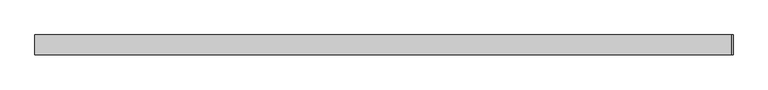
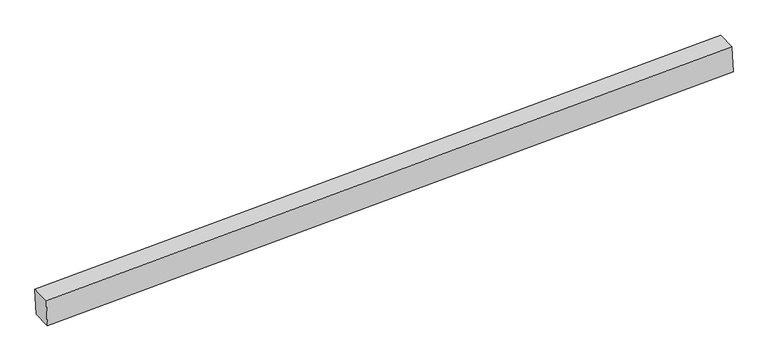
"""IFC4 building model written with IfcOpenShell, lengths in millimetres: proxy geometry, Generic Models 7:Generic Models 1:8:Generic Models 1:8 : Generic Models 7:Generic Models 1:337419:34 : Generic Models 7:Generic Models 1:8:Generic Models 1:8 : Generic Models 7:Generic Models 1:337419:315935."""

from ifc_helpers import new_model, si_unit, frame, origin, place, context, project, spatial, polyline, outline, extrude, source, transform, mapped, element, save


def generic_models_ad95f035(model_context):
    return source(origin(), model_context, "Body", "SweptSolid", [
        extrude(outline(polyline([(0.0, -4876.7999999), (0.0, 0.0), (139.7, 0.0), (139.7, -4876.7999999), (0.0, -4876.7999999)])), frame((558242.3707258, -578791.1413841, 3632.6295417), z_axis=(-0.04163054470793559, 0.0, 0.9991330730925289), x_axis=(0.0, 1.0, 0.0)), (0.0, 0.0, 1.0), 190.5),
    ])


if __name__ == "__main__":
    model = new_model("IFC4")
    model_context = context("Model", 3, world=origin())
    ifc_project = project(units=[si_unit("LENGTHUNIT", "METRE", prefix="MILLI")], contexts=[model_context])
    site = spatial("IfcSite", under=ifc_project)
    building = spatial("IfcBuilding", under=site)
    placement = place(None, origin())
    generic_models_shape = generic_models_ad95f035(model_context)
    element("IfcBuildingElementProxy", 1, Name="Generic Models 7:Generic Models 1:8:Generic Models 1:8 : Generic Models 7:Generic Models 1:337419:34 : Generic Models 7:Generic Models 1:8:Generic Models 1:8 : Generic Models 7:Generic Models 1:337419:315935", ObjectType="Generic Models 7:Generic Models 1:8:Generic Models 1:8 : Generic Models 7:Generic Models 1:337419:34 : Generic Models 7:Generic Models 1:8:Generic Models 1:8 : Generic Models 7:Generic Models 1:337419:315935", at=placement, inside=building, context=model_context, shape_type="MappedRepresentation", body=[
        mapped(generic_models_shape, transform((0.0, 0.0, 0.0), x_axis=(1.0, 0.0, 0.0), y_axis=(0.0, 1.0, 0.0), z_axis=(0.0, 0.0, 1.0))),
    ])
    save(model, "model.ifc")

# Revit data of these elements
# Type "Generic Models 7:Generic Models 1:8:Generic Models 1:8 : Generic Models 7:Generic Models 1:337419:34 : Generic Models 7:Generic Models 1:8:Generic Models 1:8 : Generic Models 7:Generic Models 1:337419:315935"
#   NameOverride = "Generic Models 7:Generic Models 1:8:Generic Models 1:8 : Generic Models 7:Generic Models 1:337419:315935"
#   ObjectTypeOverride = "Generic Models 1:8 : Generic Models 7:Generic Models 1:337419"
#   Reference = "Generic Models 1"
#   Tag = "315935"
# Element 1 (IfcBuildingElementProxy, "Generic Models 7:Generic Models 1:8:Generic Models 1:8 : Generic Models 7:Generic Models 1:337419:34 : Generic Models 7:Generic Models 1:8:Generic Models 1:8 : Generic Models 7:Generic Models 1:337419:315935")
#   Materials on its faces: "5 1/8\" X 7 1/2\" EXTERIOR GRADE GLULAM BEAMS (4'- 0 1/4\" O.C.)"
# Materials
#   "5 1/8\" X 7 1/2\" EXTERIOR GRADE GLULAM BEAMS (4'- 0 1/4\" O.C.)": class "Wood", colour RGB 183 134 68, transparency 0, Keynote = "M06181300.01", Description = "Pinus Echinata", Cost = 0
